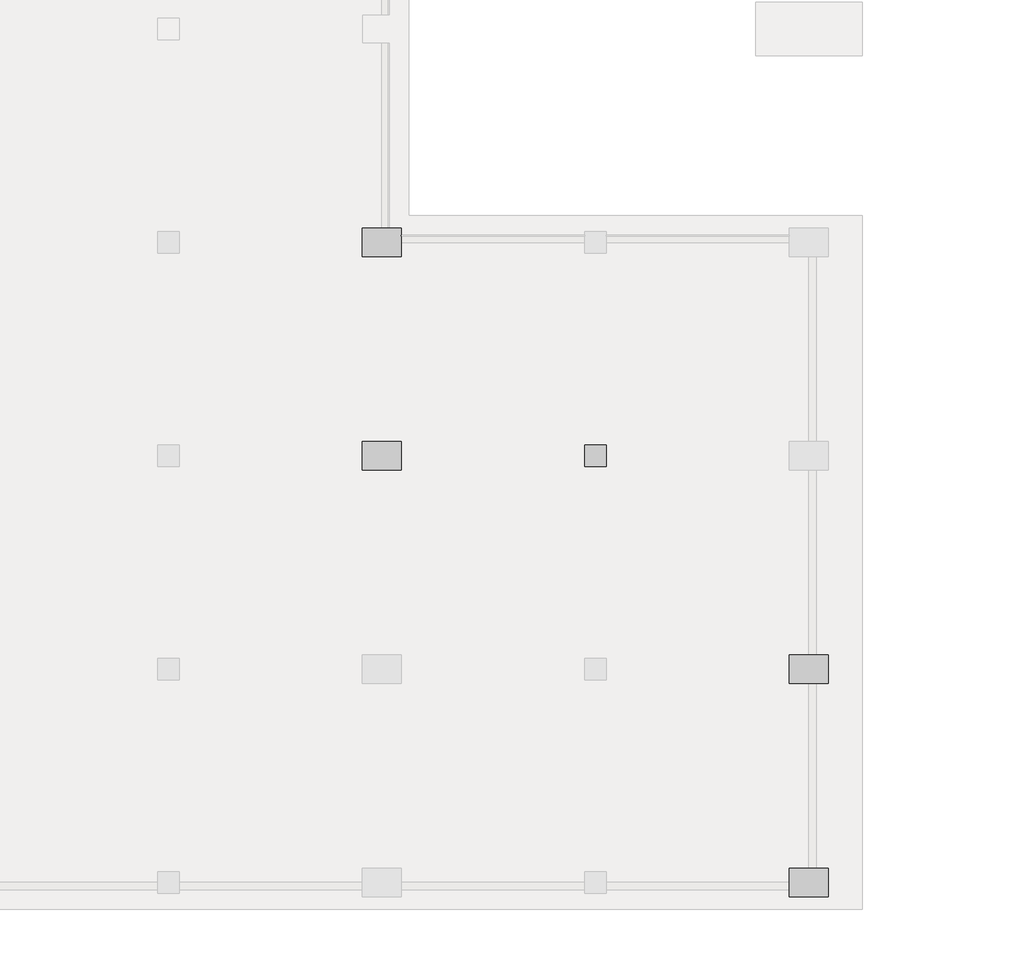
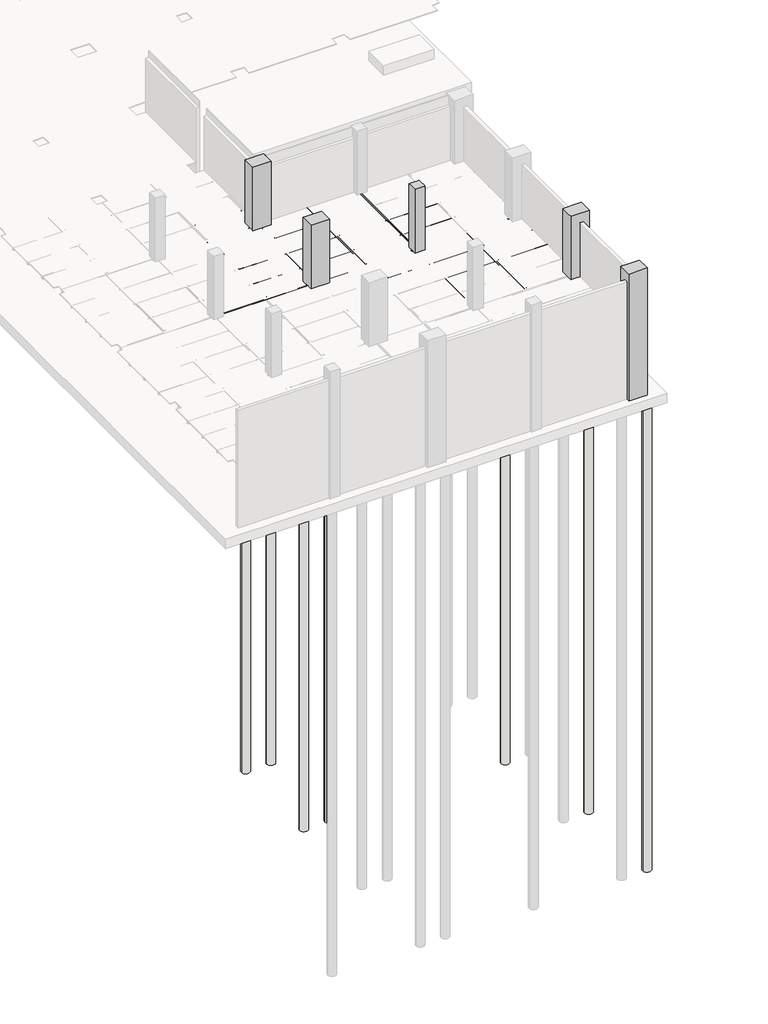
# Not in any storey, part 5 of 16: 26 beams, 7 slabs, 5 columns.
"""IFC4 building model written with IfcOpenShell, lengths in millimetres."""

from ifc_helpers import new_model, si_unit, point, frame, frame_2d, origin, place, context, project, spatial, polyline, circle_curve, trimmed, segment, composite_curve, outline, extrude, faceted_brep, element, save

model = new_model("IFC4")

# Units and contexts
model_context = context("Model", 3, world=origin())
ifc_project = project(units=[si_unit("LENGTHUNIT", "METRE", prefix="MILLI")], contexts=[model_context])

# Site, building
site = spatial("IfcSite", under=ifc_project)
building = spatial("IfcBuilding", under=site)

# Beams
placement = place(None, origin())
element("IfcBeam", 1, ObjectType="Steel Framing_H_KS : H_SB_AR_S02_H-400x200x8x13_BSG1", at=placement, inside=building, context=model_context, shape_type="SweptSolid", body=[
    extrude(outline(composite_curve([segment(polyline([(-47900.0, -4187.0381366), (-47900.0, -4200.0381366), (-48100.0, -4200.0381366), (-48100.0, -4187.0381366), (-48020.0, -4187.0381366)]), True, "CONTINUOUS"), segment(trimmed(circle_curve(frame_2d((-48020.0, -4171.0381366)), 16.0), [point((-48020.0, -4187.0381366))], [point((-48004.0, -4171.0381366))], True, "CARTESIAN"), True, "CONTINUOUS"), segment(polyline([(-48004.0, -4171.0381366), (-48004.0, -3829.0381366)]), True, "CONTINUOUS"), segment(trimmed(circle_curve(frame_2d((-48020.0, -3829.0381366)), 16.0), [point((-48004.0, -3829.0381366))], [point((-48020.0, -3813.0381366))], True, "CARTESIAN"), True, "CONTINUOUS"), segment(polyline([(-48020.0, -3813.0381366), (-48100.0, -3813.0381366), (-48100.0, -3800.0381366), (-47900.0, -3800.0381366), (-47900.0, -3813.0381366), (-47980.0, -3813.0381366)]), True, "CONTINUOUS"), segment(trimmed(circle_curve(frame_2d((-47980.0, -3829.0381366)), 16.0), [point((-47980.0, -3813.0381366))], [point((-47996.0, -3829.0381366))], True, "CARTESIAN"), True, "CONTINUOUS"), segment(polyline([(-47996.0, -3829.0381366), (-47996.0, -4171.0381366)]), True, "CONTINUOUS"), segment(trimmed(circle_curve(frame_2d((-47980.0, -4171.0381366)), 16.0), [point((-47996.0, -4171.0381366))], [point((-47980.0, -4187.0381366))], True, "CARTESIAN"), True, "CONTINUOUS"), segment(polyline([(-47980.0, -4187.0381366), (-47900.0, -4187.0381366)]), True, "CONTINUOUS")], self_intersect=False)), frame((30312.7, 0.0, 0.0), z_axis=(1.0, 0.0, 0.0), x_axis=(0.0, 1.0, 0.0)), (0.0, 0.0, 1.0), 5124.6),
])
element("IfcBeam", 2, ObjectType="Steel Framing_H_KS : H_SB_AR_S02_H-400x200x8x13_BSG2", at=placement, inside=building, context=model_context, shape_type="SweptSolid", body=[
    extrude(outline(composite_curve([segment(polyline([(-4187.0381366, 35900.0), (-4200.0381366, 35900.0), (-4200.0381366, 36100.0), (-4187.0381366, 36100.0), (-4187.0381366, 36020.0)]), True, "CONTINUOUS"), segment(trimmed(circle_curve(frame_2d((-4171.0381366, 36020.0)), 16.0), [point((-4187.0381366, 36020.0))], [point((-4171.0381366, 36004.0))], True, "CARTESIAN"), True, "CONTINUOUS"), segment(polyline([(-4171.0381366, 36004.0), (-3829.0381366, 36004.0)]), True, "CONTINUOUS"), segment(trimmed(circle_curve(frame_2d((-3829.0381366, 36020.0)), 16.0), [point((-3829.0381366, 36004.0))], [point((-3813.0381366, 36020.0))], True, "CARTESIAN"), True, "CONTINUOUS"), segment(polyline([(-3813.0381366, 36020.0), (-3813.0381366, 36100.0), (-3800.0381366, 36100.0), (-3800.0381366, 35900.0), (-3813.0381366, 35900.0), (-3813.0381366, 35980.0)]), True, "CONTINUOUS"), segment(trimmed(circle_curve(frame_2d((-3829.0381366, 35980.0)), 16.0), [point((-3813.0381366, 35980.0))], [point((-3829.0381366, 35996.0))], True, "CARTESIAN"), True, "CONTINUOUS"), segment(polyline([(-3829.0381366, 35996.0), (-4171.0381366, 35996.0)]), True, "CONTINUOUS"), segment(trimmed(circle_curve(frame_2d((-4171.0381366, 35980.0)), 16.0), [point((-4171.0381366, 35996.0))], [point((-4187.0381366, 35980.0))], True, "CARTESIAN"), True, "CONTINUOUS"), segment(polyline([(-4187.0381366, 35980.0), (-4187.0381366, 35900.0)]), True, "CONTINUOUS")], self_intersect=False)), frame((0.0, -47587.3, 0.0), z_axis=(0.0, 1.0, 0.0), x_axis=(0.0, 0.0, 1.0)), (0.0, 0.0, 1.0), 5174.6),
])
element("IfcBeam", 3, ObjectType="Steel Framing_H_KS : H_SB_AR_S02_H-400x200x8x13_BSB1", at=placement, inside=building, context=model_context, shape_type="SweptSolid", body=[
    extrude(outline(composite_curve([segment(polyline([(-4187.0381366, 32900.0), (-4200.0381366, 32900.0), (-4200.0381366, 33100.0), (-4187.0381366, 33100.0), (-4187.0381366, 33020.0)]), True, "CONTINUOUS"), segment(trimmed(circle_curve(frame_2d((-4171.0381366, 33020.0)), 16.0), [point((-4187.0381366, 33020.0))], [point((-4171.0381366, 33004.0))], True, "CARTESIAN"), True, "CONTINUOUS"), segment(polyline([(-4171.0381366, 33004.0), (-3829.0381366, 33004.0)]), True, "CONTINUOUS"), segment(trimmed(circle_curve(frame_2d((-3829.0381366, 33020.0)), 16.0), [point((-3829.0381366, 33004.0))], [point((-3813.0381366, 33020.0))], True, "CARTESIAN"), True, "CONTINUOUS"), segment(polyline([(-3813.0381366, 33020.0), (-3813.0381366, 33100.0), (-3800.0381366, 33100.0), (-3800.0381366, 32900.0), (-3813.0381366, 32900.0), (-3813.0381366, 32980.0)]), True, "CONTINUOUS"), segment(trimmed(circle_curve(frame_2d((-3829.0381366, 32980.0)), 16.0), [point((-3813.0381366, 32980.0))], [point((-3829.0381366, 32996.0))], True, "CARTESIAN"), True, "CONTINUOUS"), segment(polyline([(-3829.0381366, 32996.0), (-4171.0381366, 32996.0)]), True, "CONTINUOUS"), segment(trimmed(circle_curve(frame_2d((-4171.0381366, 32980.0)), 16.0), [point((-4171.0381366, 32996.0))], [point((-4187.0381366, 32980.0))], True, "CARTESIAN"), True, "CONTINUOUS"), segment(polyline([(-4187.0381366, 32980.0), (-4187.0381366, 32900.0)]), True, "CONTINUOUS")], self_intersect=False)), frame((0.0, -47887.3, 0.0), z_axis=(0.0, 1.0, 0.0), x_axis=(0.0, 0.0, 1.0)), (0.0, 0.0, 1.0), 5774.6),
])
element("IfcBeam", 4, ObjectType="Steel Framing_C_KS : H_SB_AR_S02_C-150x75x6.5x10_J1", at=placement, inside=building, context=model_context, shape_type="SweptSolid", body=[
    extrude(outline(composite_curve([segment(polyline([(-44977.2, -3800.0381366), (-44977.2, -3950.0381366), (-45052.2, -3950.0381366)]), True, "CONTINUOUS"), segment(trimmed(circle_curve(frame_2d((-45042.2, -3950.0381366)), 10.0), [point((-45052.2, -3950.0381366))], [point((-45042.2, -3940.0381366))], False, "CARTESIAN"), True, "CONTINUOUS"), segment(polyline([(-45042.2, -3940.0381366), (-44983.7, -3930.7726469), (-44983.7, -3819.3036264), (-45042.2, -3810.0381366)]), True, "CONTINUOUS"), segment(trimmed(circle_curve(frame_2d((-45042.2, -3800.0381366)), 10.0), [point((-45042.2, -3810.0381366))], [point((-45052.2, -3800.0381366))], False, "CARTESIAN"), True, "CONTINUOUS"), segment(polyline([(-45052.2, -3800.0381366), (-44977.2, -3800.0381366)]), True, "CONTINUOUS")], self_intersect=False)), frame((33112.7, 0.0, 0.0), z_axis=(1.0, 0.0, 0.0), x_axis=(0.0, 1.0, 0.0)), (0.0, 0.0, 1.0), 2774.6),
])
element("IfcBeam", 5, ObjectType="Steel Framing_C_KS : H_SB_AR_S02_C-150x75x6.5x10_J1", at=placement, inside=building, context=model_context, shape_type="SweptSolid", body=[
    extrude(outline(composite_curve([segment(polyline([(-46477.2, -3800.0381366), (-46477.2, -3950.0381366), (-46552.2, -3950.0381366)]), True, "CONTINUOUS"), segment(trimmed(circle_curve(frame_2d((-46542.2, -3950.0381366)), 10.0), [point((-46552.2, -3950.0381366))], [point((-46542.2, -3940.0381366))], False, "CARTESIAN"), True, "CONTINUOUS"), segment(polyline([(-46542.2, -3940.0381366), (-46483.7, -3930.7726469), (-46483.7, -3819.3036264), (-46542.2, -3810.0381366)]), True, "CONTINUOUS"), segment(trimmed(circle_curve(frame_2d((-46542.2, -3800.0381366)), 10.0), [point((-46542.2, -3810.0381366))], [point((-46552.2, -3800.0381366))], False, "CARTESIAN"), True, "CONTINUOUS"), segment(polyline([(-46552.2, -3800.0381366), (-46477.2, -3800.0381366)]), True, "CONTINUOUS")], self_intersect=False)), frame((33112.7, 0.0, 0.0), z_axis=(1.0, 0.0, 0.0), x_axis=(0.0, 1.0, 0.0)), (0.0, 0.0, 1.0), 2774.6),
])
element("IfcBeam", 6, ObjectType="Steel Framing_C_KS : H_SB_AR_S02_C-150x75x6.5x10_J1", at=placement, inside=building, context=model_context, shape_type="SweptSolid", body=[
    extrude(outline(composite_curve([segment(polyline([(-43477.2, -3800.0381366), (-43477.2, -3950.0381366), (-43552.2, -3950.0381366)]), True, "CONTINUOUS"), segment(trimmed(circle_curve(frame_2d((-43542.2, -3950.0381366)), 10.0), [point((-43552.2, -3950.0381366))], [point((-43542.2, -3940.0381366))], False, "CARTESIAN"), True, "CONTINUOUS"), segment(polyline([(-43542.2, -3940.0381366), (-43483.7, -3930.7726469), (-43483.7, -3819.3036264), (-43542.2, -3810.0381366)]), True, "CONTINUOUS"), segment(trimmed(circle_curve(frame_2d((-43542.2, -3800.0381366)), 10.0), [point((-43542.2, -3810.0381366))], [point((-43552.2, -3800.0381366))], False, "CARTESIAN"), True, "CONTINUOUS"), segment(polyline([(-43552.2, -3800.0381366), (-43477.2, -3800.0381366)]), True, "CONTINUOUS")], self_intersect=False)), frame((33112.7, 0.0, 0.0), z_axis=(1.0, 0.0, 0.0), x_axis=(0.0, 1.0, 0.0)), (0.0, 0.0, 1.0), 2774.6),
])
element("IfcBeam", 7, ObjectType="Steel Framing_H_KS : H_SB_AR_S02_H-400x200x8x13_BSG1", at=placement, inside=building, context=model_context, shape_type="SweptSolid", body=[
    extrude(outline(composite_curve([segment(polyline([(-47900.0, -4187.0381366), (-47900.0, -4200.0381366), (-48100.0, -4200.0381366), (-48100.0, -4187.0381366), (-48020.0, -4187.0381366)]), True, "CONTINUOUS"), segment(trimmed(circle_curve(frame_2d((-48020.0, -4171.0381366)), 16.0), [point((-48020.0, -4187.0381366))], [point((-48004.0, -4171.0381366))], True, "CARTESIAN"), True, "CONTINUOUS"), segment(polyline([(-48004.0, -4171.0381366), (-48004.0, -3829.0381366)]), True, "CONTINUOUS"), segment(trimmed(circle_curve(frame_2d((-48020.0, -3829.0381366)), 16.0), [point((-48004.0, -3829.0381366))], [point((-48020.0, -3813.0381366))], True, "CARTESIAN"), True, "CONTINUOUS"), segment(polyline([(-48020.0, -3813.0381366), (-48100.0, -3813.0381366), (-48100.0, -3800.0381366), (-47900.0, -3800.0381366), (-47900.0, -3813.0381366), (-47980.0, -3813.0381366)]), True, "CONTINUOUS"), segment(trimmed(circle_curve(frame_2d((-47980.0, -3829.0381366)), 16.0), [point((-47980.0, -3813.0381366))], [point((-47996.0, -3829.0381366))], True, "CARTESIAN"), True, "CONTINUOUS"), segment(polyline([(-47996.0, -3829.0381366), (-47996.0, -4171.0381366)]), True, "CONTINUOUS"), segment(trimmed(circle_curve(frame_2d((-47980.0, -4171.0381366)), 16.0), [point((-47996.0, -4171.0381366))], [point((-47980.0, -4187.0381366))], True, "CARTESIAN"), True, "CONTINUOUS"), segment(polyline([(-47980.0, -4187.0381366), (-47900.0, -4187.0381366)]), True, "CONTINUOUS")], self_intersect=False)), frame((36562.7, 0.0, 0.0), z_axis=(1.0, 0.0, 0.0), x_axis=(0.0, 1.0, 0.0)), (0.0, 0.0, 1.0), 5124.6),
])
element("IfcBeam", 8, ObjectType="Steel Framing_H_KS : H_SB_AR_S02_H-400x200x8x13_BSG2", at=placement, inside=building, context=model_context, shape_type="SweptSolid", body=[
    extrude(outline(composite_curve([segment(polyline([(-4187.0381366, 41900.0), (-4200.0381366, 41900.0), (-4200.0381366, 42100.0), (-4187.0381366, 42100.0), (-4187.0381366, 42020.0)]), True, "CONTINUOUS"), segment(trimmed(circle_curve(frame_2d((-4171.0381366, 42020.0)), 16.0), [point((-4187.0381366, 42020.0))], [point((-4171.0381366, 42004.0))], True, "CARTESIAN"), True, "CONTINUOUS"), segment(polyline([(-4171.0381366, 42004.0), (-3829.0381366, 42004.0)]), True, "CONTINUOUS"), segment(trimmed(circle_curve(frame_2d((-3829.0381366, 42020.0)), 16.0), [point((-3829.0381366, 42004.0))], [point((-3813.0381366, 42020.0))], True, "CARTESIAN"), True, "CONTINUOUS"), segment(polyline([(-3813.0381366, 42020.0), (-3813.0381366, 42100.0), (-3800.0381366, 42100.0), (-3800.0381366, 41900.0), (-3813.0381366, 41900.0), (-3813.0381366, 41980.0)]), True, "CONTINUOUS"), segment(trimmed(circle_curve(frame_2d((-3829.0381366, 41980.0)), 16.0), [point((-3813.0381366, 41980.0))], [point((-3829.0381366, 41996.0))], True, "CARTESIAN"), True, "CONTINUOUS"), segment(polyline([(-3829.0381366, 41996.0), (-4171.0381366, 41996.0)]), True, "CONTINUOUS"), segment(trimmed(circle_curve(frame_2d((-4171.0381366, 41980.0)), 16.0), [point((-4171.0381366, 41996.0))], [point((-4187.0381366, 41980.0))], True, "CARTESIAN"), True, "CONTINUOUS"), segment(polyline([(-4187.0381366, 41980.0), (-4187.0381366, 41900.0)]), True, "CONTINUOUS")], self_intersect=False)), frame((0.0, -47687.3, 0.0), z_axis=(0.0, 1.0, 0.0), x_axis=(0.0, 0.0, 1.0)), (0.0, 0.0, 1.0), 5374.6),
])
element("IfcBeam", 9, ObjectType="Steel Framing_H_KS : H_SB_AR_S02_H-400x200x8x13_BSB1", at=placement, inside=building, context=model_context, shape_type="SweptSolid", body=[
    extrude(outline(composite_curve([segment(polyline([(-4187.0381366, 38900.0), (-4200.0381366, 38900.0), (-4200.0381366, 39100.0), (-4187.0381366, 39100.0), (-4187.0381366, 39020.0)]), True, "CONTINUOUS"), segment(trimmed(circle_curve(frame_2d((-4171.0381366, 39020.0)), 16.0), [point((-4187.0381366, 39020.0))], [point((-4171.0381366, 39004.0))], True, "CARTESIAN"), True, "CONTINUOUS"), segment(polyline([(-4171.0381366, 39004.0), (-3829.0381366, 39004.0)]), True, "CONTINUOUS"), segment(trimmed(circle_curve(frame_2d((-3829.0381366, 39020.0)), 16.0), [point((-3829.0381366, 39004.0))], [point((-3813.0381366, 39020.0))], True, "CARTESIAN"), True, "CONTINUOUS"), segment(polyline([(-3813.0381366, 39020.0), (-3813.0381366, 39100.0), (-3800.0381366, 39100.0), (-3800.0381366, 38900.0), (-3813.0381366, 38900.0), (-3813.0381366, 38980.0)]), True, "CONTINUOUS"), segment(trimmed(circle_curve(frame_2d((-3829.0381366, 38980.0)), 16.0), [point((-3813.0381366, 38980.0))], [point((-3829.0381366, 38996.0))], True, "CARTESIAN"), True, "CONTINUOUS"), segment(polyline([(-3829.0381366, 38996.0), (-4171.0381366, 38996.0)]), True, "CONTINUOUS"), segment(trimmed(circle_curve(frame_2d((-4171.0381366, 38980.0)), 16.0), [point((-4171.0381366, 38996.0))], [point((-4187.0381366, 38980.0))], True, "CARTESIAN"), True, "CONTINUOUS"), segment(polyline([(-4187.0381366, 38980.0), (-4187.0381366, 38900.0)]), True, "CONTINUOUS")], self_intersect=False)), frame((0.0, -47887.3, 0.0), z_axis=(0.0, 1.0, 0.0), x_axis=(0.0, 0.0, 1.0)), (0.0, 0.0, 1.0), 5887.3),
])
element("IfcBeam", 10, ObjectType="Steel Framing_C_KS : H_SB_AR_S02_C-150x75x6.5x10_J1", at=placement, inside=building, context=model_context, shape_type="SweptSolid", body=[
    extrude(outline(composite_curve([segment(polyline([(-44977.2, -3800.0381366), (-44977.2, -3950.0381366), (-45052.2, -3950.0381366)]), True, "CONTINUOUS"), segment(trimmed(circle_curve(frame_2d((-45042.2, -3950.0381366)), 10.0), [point((-45052.2, -3950.0381366))], [point((-45042.2, -3940.0381366))], False, "CARTESIAN"), True, "CONTINUOUS"), segment(polyline([(-45042.2, -3940.0381366), (-44983.7, -3930.7726469), (-44983.7, -3819.3036264), (-45042.2, -3810.0381366)]), True, "CONTINUOUS"), segment(trimmed(circle_curve(frame_2d((-45042.2, -3800.0381366)), 10.0), [point((-45042.2, -3810.0381366))], [point((-45052.2, -3800.0381366))], False, "CARTESIAN"), True, "CONTINUOUS"), segment(polyline([(-45052.2, -3800.0381366), (-44977.2, -3800.0381366)]), True, "CONTINUOUS")], self_intersect=False)), frame((36112.7, 0.0, 0.0), z_axis=(1.0, 0.0, 0.0), x_axis=(0.0, 1.0, 0.0)), (0.0, 0.0, 1.0), 2774.6),
])
element("IfcBeam", 11, ObjectType="Steel Framing_C_KS : H_SB_AR_S02_C-150x75x6.5x10_J1", at=placement, inside=building, context=model_context, shape_type="SweptSolid", body=[
    extrude(outline(composite_curve([segment(polyline([(-46477.2, -3800.0381366), (-46477.2, -3950.0381366), (-46552.2, -3950.0381366)]), True, "CONTINUOUS"), segment(trimmed(circle_curve(frame_2d((-46542.2, -3950.0381366)), 10.0), [point((-46552.2, -3950.0381366))], [point((-46542.2, -3940.0381366))], False, "CARTESIAN"), True, "CONTINUOUS"), segment(polyline([(-46542.2, -3940.0381366), (-46483.7, -3930.7726469), (-46483.7, -3819.3036264), (-46542.2, -3810.0381366)]), True, "CONTINUOUS"), segment(trimmed(circle_curve(frame_2d((-46542.2, -3800.0381366)), 10.0), [point((-46542.2, -3810.0381366))], [point((-46552.2, -3800.0381366))], False, "CARTESIAN"), True, "CONTINUOUS"), segment(polyline([(-46552.2, -3800.0381366), (-46477.2, -3800.0381366)]), True, "CONTINUOUS")], self_intersect=False)), frame((36112.7, 0.0, 0.0), z_axis=(1.0, 0.0, 0.0), x_axis=(0.0, 1.0, 0.0)), (0.0, 0.0, 1.0), 2774.6),
])
element("IfcBeam", 12, ObjectType="Steel Framing_C_KS : H_SB_AR_S02_C-150x75x6.5x10_J1", at=placement, inside=building, context=model_context, shape_type="SweptSolid", body=[
    extrude(outline(composite_curve([segment(polyline([(-43477.2, -3800.0381366), (-43477.2, -3950.0381366), (-43552.2, -3950.0381366)]), True, "CONTINUOUS"), segment(trimmed(circle_curve(frame_2d((-43542.2, -3950.0381366)), 10.0), [point((-43552.2, -3950.0381366))], [point((-43542.2, -3940.0381366))], False, "CARTESIAN"), True, "CONTINUOUS"), segment(polyline([(-43542.2, -3940.0381366), (-43483.7, -3930.7726469), (-43483.7, -3819.3036264), (-43542.2, -3810.0381366)]), True, "CONTINUOUS"), segment(trimmed(circle_curve(frame_2d((-43542.2, -3800.0381366)), 10.0), [point((-43542.2, -3810.0381366))], [point((-43552.2, -3800.0381366))], False, "CARTESIAN"), True, "CONTINUOUS"), segment(polyline([(-43552.2, -3800.0381366), (-43477.2, -3800.0381366)]), True, "CONTINUOUS")], self_intersect=False)), frame((36112.7, 0.0, 0.0), z_axis=(1.0, 0.0, 0.0), x_axis=(0.0, 1.0, 0.0)), (0.0, 0.0, 1.0), 2774.6),
])
element("IfcBeam", 13, ObjectType="Steel Framing_C_KS : H_SB_AR_S02_C-150x75x6.5x10_J1", at=placement, inside=building, context=model_context, shape_type="SweptSolid", body=[
    extrude(outline(composite_curve([segment(polyline([(-44977.2, -3800.0381366), (-44977.2, -3950.0381366), (-45052.2, -3950.0381366)]), True, "CONTINUOUS"), segment(trimmed(circle_curve(frame_2d((-45042.2, -3950.0381366)), 10.0), [point((-45052.2, -3950.0381366))], [point((-45042.2, -3940.0381366))], False, "CARTESIAN"), True, "CONTINUOUS"), segment(polyline([(-45042.2, -3940.0381366), (-44983.7, -3930.7726469), (-44983.7, -3819.3036264), (-45042.2, -3810.0381366)]), True, "CONTINUOUS"), segment(trimmed(circle_curve(frame_2d((-45042.2, -3800.0381366)), 10.0), [point((-45042.2, -3810.0381366))], [point((-45052.2, -3800.0381366))], False, "CARTESIAN"), True, "CONTINUOUS"), segment(polyline([(-45052.2, -3800.0381366), (-44977.2, -3800.0381366)]), True, "CONTINUOUS")], self_intersect=False)), frame((39112.7, 0.0, 0.0), z_axis=(1.0, 0.0, 0.0), x_axis=(0.0, 1.0, 0.0)), (0.0, 0.0, 1.0), 2774.6),
])
element("IfcBeam", 14, ObjectType="Steel Framing_C_KS : H_SB_AR_S02_C-150x75x6.5x10_J1", at=placement, inside=building, context=model_context, shape_type="SweptSolid", body=[
    extrude(outline(composite_curve([segment(polyline([(-46477.2, -3800.0381366), (-46477.2, -3950.0381366), (-46552.2, -3950.0381366)]), True, "CONTINUOUS"), segment(trimmed(circle_curve(frame_2d((-46542.2, -3950.0381366)), 10.0), [point((-46552.2, -3950.0381366))], [point((-46542.2, -3940.0381366))], False, "CARTESIAN"), True, "CONTINUOUS"), segment(polyline([(-46542.2, -3940.0381366), (-46483.7, -3930.7726469), (-46483.7, -3819.3036264), (-46542.2, -3810.0381366)]), True, "CONTINUOUS"), segment(trimmed(circle_curve(frame_2d((-46542.2, -3800.0381366)), 10.0), [point((-46542.2, -3810.0381366))], [point((-46552.2, -3800.0381366))], False, "CARTESIAN"), True, "CONTINUOUS"), segment(polyline([(-46552.2, -3800.0381366), (-46477.2, -3800.0381366)]), True, "CONTINUOUS")], self_intersect=False)), frame((39112.7, 0.0, 0.0), z_axis=(1.0, 0.0, 0.0), x_axis=(0.0, 1.0, 0.0)), (0.0, 0.0, 1.0), 2774.6),
])
element("IfcBeam", 15, ObjectType="Steel Framing_H_KS : H_SB_AR_S02_H-400x200x8x13_BSG1", at=placement, inside=building, context=model_context, shape_type="SweptSolid", body=[
    extrude(outline(composite_curve([segment(polyline([(-47900.0, -4187.0381366), (-47900.0, -4200.0381366), (-48100.0, -4200.0381366), (-48100.0, -4187.0381366), (-48020.0, -4187.0381366)]), True, "CONTINUOUS"), segment(trimmed(circle_curve(frame_2d((-48020.0, -4171.0381366)), 16.0), [point((-48020.0, -4187.0381366))], [point((-48004.0, -4171.0381366))], True, "CARTESIAN"), True, "CONTINUOUS"), segment(polyline([(-48004.0, -4171.0381366), (-48004.0, -3829.0381366)]), True, "CONTINUOUS"), segment(trimmed(circle_curve(frame_2d((-48020.0, -3829.0381366)), 16.0), [point((-48004.0, -3829.0381366))], [point((-48020.0, -3813.0381366))], True, "CARTESIAN"), True, "CONTINUOUS"), segment(polyline([(-48020.0, -3813.0381366), (-48100.0, -3813.0381366), (-48100.0, -3800.0381366), (-47900.0, -3800.0381366), (-47900.0, -3813.0381366), (-47980.0, -3813.0381366)]), True, "CONTINUOUS"), segment(trimmed(circle_curve(frame_2d((-47980.0, -3829.0381366)), 16.0), [point((-47980.0, -3813.0381366))], [point((-47996.0, -3829.0381366))], True, "CARTESIAN"), True, "CONTINUOUS"), segment(polyline([(-47996.0, -3829.0381366), (-47996.0, -4171.0381366)]), True, "CONTINUOUS"), segment(trimmed(circle_curve(frame_2d((-47980.0, -4171.0381366)), 16.0), [point((-47996.0, -4171.0381366))], [point((-47980.0, -4187.0381366))], True, "CARTESIAN"), True, "CONTINUOUS"), segment(polyline([(-47980.0, -4187.0381366), (-47900.0, -4187.0381366)]), True, "CONTINUOUS")], self_intersect=False)), frame((42312.7, 0.0, 0.0), z_axis=(1.0, 0.0, 0.0), x_axis=(0.0, 1.0, 0.0)), (0.0, 0.0, 1.0), 5124.6),
])
element("IfcBeam", 16, ObjectType="Steel Framing_C_KS : H_SB_AR_S02_C-150x75x6.5x10_J1", at=placement, inside=building, context=model_context, shape_type="SweptSolid", body=[
    extrude(outline(composite_curve([segment(polyline([(-44977.2, -3800.0381366), (-44977.2, -3950.0381366), (-45052.2, -3950.0381366)]), True, "CONTINUOUS"), segment(trimmed(circle_curve(frame_2d((-45042.2, -3950.0381366)), 10.0), [point((-45052.2, -3950.0381366))], [point((-45042.2, -3940.0381366))], False, "CARTESIAN"), True, "CONTINUOUS"), segment(polyline([(-45042.2, -3940.0381366), (-44983.7, -3930.7726469), (-44983.7, -3819.3036264), (-45042.2, -3810.0381366)]), True, "CONTINUOUS"), segment(trimmed(circle_curve(frame_2d((-45042.2, -3800.0381366)), 10.0), [point((-45042.2, -3810.0381366))], [point((-45052.2, -3800.0381366))], False, "CARTESIAN"), True, "CONTINUOUS"), segment(polyline([(-45052.2, -3800.0381366), (-44977.2, -3800.0381366)]), True, "CONTINUOUS")], self_intersect=False)), frame((42112.7, 0.0, 0.0), z_axis=(1.0, 0.0, 0.0), x_axis=(0.0, 1.0, 0.0)), (0.0, 0.0, 1.0), 2774.6),
])
element("IfcBeam", 17, ObjectType="Steel Framing_C_KS : H_SB_AR_S02_C-150x75x6.5x10_J1", at=placement, inside=building, context=model_context, shape_type="SweptSolid", body=[
    extrude(outline(composite_curve([segment(polyline([(-46477.2, -3800.0381366), (-46477.2, -3950.0381366), (-46552.2, -3950.0381366)]), True, "CONTINUOUS"), segment(trimmed(circle_curve(frame_2d((-46542.2, -3950.0381366)), 10.0), [point((-46552.2, -3950.0381366))], [point((-46542.2, -3940.0381366))], False, "CARTESIAN"), True, "CONTINUOUS"), segment(polyline([(-46542.2, -3940.0381366), (-46483.7, -3930.7726469), (-46483.7, -3819.3036264), (-46542.2, -3810.0381366)]), True, "CONTINUOUS"), segment(trimmed(circle_curve(frame_2d((-46542.2, -3800.0381366)), 10.0), [point((-46542.2, -3810.0381366))], [point((-46552.2, -3800.0381366))], False, "CARTESIAN"), True, "CONTINUOUS"), segment(polyline([(-46552.2, -3800.0381366), (-46477.2, -3800.0381366)]), True, "CONTINUOUS")], self_intersect=False)), frame((42112.7, 0.0, 0.0), z_axis=(1.0, 0.0, 0.0), x_axis=(0.0, 1.0, 0.0)), (0.0, 0.0, 1.0), 2774.6),
])
element("IfcBeam", 18, ObjectType="Steel Framing_H_KS : H_SB_AR_S02_H-400x200x8x13_BSG2", at=placement, inside=building, context=model_context, shape_type="SweptSolid", body=[
    extrude(outline(composite_curve([segment(polyline([(-4187.0381366, 41900.0), (-4200.0381366, 41900.0), (-4200.0381366, 42100.0), (-4187.0381366, 42100.0), (-4187.0381366, 42020.0)]), True, "CONTINUOUS"), segment(trimmed(circle_curve(frame_2d((-4171.0381366, 42020.0)), 16.0), [point((-4187.0381366, 42020.0))], [point((-4171.0381366, 42004.0))], True, "CARTESIAN"), True, "CONTINUOUS"), segment(polyline([(-4171.0381366, 42004.0), (-3829.0381366, 42004.0)]), True, "CONTINUOUS"), segment(trimmed(circle_curve(frame_2d((-3829.0381366, 42020.0)), 16.0), [point((-3829.0381366, 42004.0))], [point((-3813.0381366, 42020.0))], True, "CARTESIAN"), True, "CONTINUOUS"), segment(polyline([(-3813.0381366, 42020.0), (-3813.0381366, 42100.0), (-3800.0381366, 42100.0), (-3800.0381366, 41900.0), (-3813.0381366, 41900.0), (-3813.0381366, 41980.0)]), True, "CONTINUOUS"), segment(trimmed(circle_curve(frame_2d((-3829.0381366, 41980.0)), 16.0), [point((-3813.0381366, 41980.0))], [point((-3829.0381366, 41996.0))], True, "CARTESIAN"), True, "CONTINUOUS"), segment(polyline([(-3829.0381366, 41996.0), (-4171.0381366, 41996.0)]), True, "CONTINUOUS"), segment(trimmed(circle_curve(frame_2d((-4171.0381366, 41980.0)), 16.0), [point((-4171.0381366, 41996.0))], [point((-4187.0381366, 41980.0))], True, "CARTESIAN"), True, "CONTINUOUS"), segment(polyline([(-4187.0381366, 41980.0), (-4187.0381366, 41900.0)]), True, "CONTINUOUS")], self_intersect=False)), frame((0.0, -53687.3, 0.0), z_axis=(0.0, 1.0, 0.0), x_axis=(0.0, 0.0, 1.0)), (0.0, 0.0, 1.0), 5374.6),
])
element("IfcBeam", 19, ObjectType="Steel Framing_C_KS : H_SB_AR_S02_C-150x75x6.5x10_J1", at=placement, inside=building, context=model_context, shape_type="SweptSolid", body=[
    extrude(outline(composite_curve([segment(polyline([(-49477.2, -3800.0381366), (-49477.2, -3950.0381366), (-49552.2, -3950.0381366)]), True, "CONTINUOUS"), segment(trimmed(circle_curve(frame_2d((-49542.2, -3950.0381366)), 10.0), [point((-49552.2, -3950.0381366))], [point((-49542.2, -3940.0381366))], False, "CARTESIAN"), True, "CONTINUOUS"), segment(polyline([(-49542.2, -3940.0381366), (-49483.7, -3930.7726469), (-49483.7, -3819.3036264), (-49542.2, -3810.0381366)]), True, "CONTINUOUS"), segment(trimmed(circle_curve(frame_2d((-49542.2, -3800.0381366)), 10.0), [point((-49542.2, -3810.0381366))], [point((-49552.2, -3800.0381366))], False, "CARTESIAN"), True, "CONTINUOUS"), segment(polyline([(-49552.2, -3800.0381366), (-49477.2, -3800.0381366)]), True, "CONTINUOUS")], self_intersect=False)), frame((39112.7, 0.0, 0.0), z_axis=(1.0, 0.0, 0.0), x_axis=(0.0, 1.0, 0.0)), (0.0, 0.0, 1.0), 2774.6),
])
element("IfcBeam", 20, ObjectType="Steel Framing_H_KS : H_SB_AR_S02_H-400x200x8x13_BSB1", at=placement, inside=building, context=model_context, shape_type="SweptSolid", body=[
    extrude(outline(composite_curve([segment(polyline([(-4187.0381366, 44900.0), (-4200.0381366, 44900.0), (-4200.0381366, 45100.0), (-4187.0381366, 45100.0), (-4187.0381366, 45020.0)]), True, "CONTINUOUS"), segment(trimmed(circle_curve(frame_2d((-4171.0381366, 45020.0)), 16.0), [point((-4187.0381366, 45020.0))], [point((-4171.0381366, 45004.0))], True, "CARTESIAN"), True, "CONTINUOUS"), segment(polyline([(-4171.0381366, 45004.0), (-3829.0381366, 45004.0)]), True, "CONTINUOUS"), segment(trimmed(circle_curve(frame_2d((-3829.0381366, 45020.0)), 16.0), [point((-3829.0381366, 45004.0))], [point((-3813.0381366, 45020.0))], True, "CARTESIAN"), True, "CONTINUOUS"), segment(polyline([(-3813.0381366, 45020.0), (-3813.0381366, 45100.0), (-3800.0381366, 45100.0), (-3800.0381366, 44900.0), (-3813.0381366, 44900.0), (-3813.0381366, 44980.0)]), True, "CONTINUOUS"), segment(trimmed(circle_curve(frame_2d((-3829.0381366, 44980.0)), 16.0), [point((-3813.0381366, 44980.0))], [point((-3829.0381366, 44996.0))], True, "CARTESIAN"), True, "CONTINUOUS"), segment(polyline([(-3829.0381366, 44996.0), (-4171.0381366, 44996.0)]), True, "CONTINUOUS"), segment(trimmed(circle_curve(frame_2d((-4171.0381366, 44980.0)), 16.0), [point((-4171.0381366, 44996.0))], [point((-4187.0381366, 44980.0))], True, "CARTESIAN"), True, "CONTINUOUS"), segment(polyline([(-4187.0381366, 44980.0), (-4187.0381366, 44900.0)]), True, "CONTINUOUS")], self_intersect=False)), frame((0.0, -53887.3, 0.0), z_axis=(0.0, 1.0, 0.0), x_axis=(0.0, 0.0, 1.0)), (0.0, 0.0, 1.0), 5774.6),
])
element("IfcBeam", 21, ObjectType="Steel Framing_C_KS : H_SB_AR_S02_C-150x75x6.5x10_J1", at=placement, inside=building, context=model_context, shape_type="SweptSolid", body=[
    extrude(outline(composite_curve([segment(polyline([(-50977.2, -3800.0381366), (-50977.2, -3950.0381366), (-51052.2, -3950.0381366)]), True, "CONTINUOUS"), segment(trimmed(circle_curve(frame_2d((-51042.2, -3950.0381366)), 10.0), [point((-51052.2, -3950.0381366))], [point((-51042.2, -3940.0381366))], False, "CARTESIAN"), True, "CONTINUOUS"), segment(polyline([(-51042.2, -3940.0381366), (-50983.7, -3930.7726469), (-50983.7, -3819.3036264), (-51042.2, -3810.0381366)]), True, "CONTINUOUS"), segment(trimmed(circle_curve(frame_2d((-51042.2, -3800.0381366)), 10.0), [point((-51042.2, -3810.0381366))], [point((-51052.2, -3800.0381366))], False, "CARTESIAN"), True, "CONTINUOUS"), segment(polyline([(-51052.2, -3800.0381366), (-50977.2, -3800.0381366)]), True, "CONTINUOUS")], self_intersect=False)), frame((42112.7, 0.0, 0.0), z_axis=(1.0, 0.0, 0.0), x_axis=(0.0, 1.0, 0.0)), (0.0, 0.0, 1.0), 2774.6),
])
element("IfcBeam", 22, ObjectType="Steel Framing_C_KS : H_SB_AR_S02_C-150x75x6.5x10_J1", at=placement, inside=building, context=model_context, shape_type="SweptSolid", body=[
    extrude(outline(composite_curve([segment(polyline([(-49477.2, -3800.0381366), (-49477.2, -3950.0381366), (-49552.2, -3950.0381366)]), True, "CONTINUOUS"), segment(trimmed(circle_curve(frame_2d((-49542.2, -3950.0381366)), 10.0), [point((-49552.2, -3950.0381366))], [point((-49542.2, -3940.0381366))], False, "CARTESIAN"), True, "CONTINUOUS"), segment(polyline([(-49542.2, -3940.0381366), (-49483.7, -3930.7726469), (-49483.7, -3819.3036264), (-49542.2, -3810.0381366)]), True, "CONTINUOUS"), segment(trimmed(circle_curve(frame_2d((-49542.2, -3800.0381366)), 10.0), [point((-49542.2, -3810.0381366))], [point((-49552.2, -3800.0381366))], False, "CARTESIAN"), True, "CONTINUOUS"), segment(polyline([(-49552.2, -3800.0381366), (-49477.2, -3800.0381366)]), True, "CONTINUOUS")], self_intersect=False)), frame((42112.7, 0.0, 0.0), z_axis=(1.0, 0.0, 0.0), x_axis=(0.0, 1.0, 0.0)), (0.0, 0.0, 1.0), 2774.6),
])
element("IfcBeam", 23, ObjectType="Steel Framing_C_KS : H_SB_AR_S02_C-150x75x6.5x10_J1", at=placement, inside=building, context=model_context, shape_type="SweptSolid", body=[
    extrude(outline(composite_curve([segment(polyline([(-50977.2, -3800.0381366), (-50977.2, -3950.0381366), (-51052.2, -3950.0381366)]), True, "CONTINUOUS"), segment(trimmed(circle_curve(frame_2d((-51042.2, -3950.0381366)), 10.0), [point((-51052.2, -3950.0381366))], [point((-51042.2, -3940.0381366))], False, "CARTESIAN"), True, "CONTINUOUS"), segment(polyline([(-51042.2, -3940.0381366), (-50983.7, -3930.7726469), (-50983.7, -3819.3036264), (-51042.2, -3810.0381366)]), True, "CONTINUOUS"), segment(trimmed(circle_curve(frame_2d((-51042.2, -3800.0381366)), 10.0), [point((-51042.2, -3810.0381366))], [point((-51052.2, -3800.0381366))], False, "CARTESIAN"), True, "CONTINUOUS"), segment(polyline([(-51052.2, -3800.0381366), (-50977.2, -3800.0381366)]), True, "CONTINUOUS")], self_intersect=False)), frame((45112.7, 0.0, 0.0), z_axis=(1.0, 0.0, 0.0), x_axis=(0.0, 1.0, 0.0)), (0.0, 0.0, 1.0), 2887.3),
])
element("IfcBeam", 24, ObjectType="Steel Framing_C_KS : H_SB_AR_S02_C-150x75x6.5x10_J1", at=placement, inside=building, context=model_context, shape_type="SweptSolid", body=[
    extrude(outline(composite_curve([segment(polyline([(-49477.2, -3800.0381366), (-49477.2, -3950.0381366), (-49552.2, -3950.0381366)]), True, "CONTINUOUS"), segment(trimmed(circle_curve(frame_2d((-49542.2, -3950.0381366)), 10.0), [point((-49552.2, -3950.0381366))], [point((-49542.2, -3940.0381366))], False, "CARTESIAN"), True, "CONTINUOUS"), segment(polyline([(-49542.2, -3940.0381366), (-49483.7, -3930.7726469), (-49483.7, -3819.3036264), (-49542.2, -3810.0381366)]), True, "CONTINUOUS"), segment(trimmed(circle_curve(frame_2d((-49542.2, -3800.0381366)), 10.0), [point((-49542.2, -3810.0381366))], [point((-49552.2, -3800.0381366))], False, "CARTESIAN"), True, "CONTINUOUS"), segment(polyline([(-49552.2, -3800.0381366), (-49477.2, -3800.0381366)]), True, "CONTINUOUS")], self_intersect=False)), frame((45112.7, 0.0, 0.0), z_axis=(1.0, 0.0, 0.0), x_axis=(0.0, 1.0, 0.0)), (0.0, 0.0, 1.0), 2887.3),
])
element("IfcBeam", 25, ObjectType="Steel Framing_H_KS : H_SB_AR_S02_H-400x200x8x13_BSG1", at=placement, inside=building, context=model_context, shape_type="SweptSolid", body=[
    extrude(outline(composite_curve([segment(polyline([(-41900.0, -4187.0381366), (-41900.0, -4200.0381366), (-42100.0, -4200.0381366), (-42100.0, -4187.0381366), (-42020.0, -4187.0381366)]), True, "CONTINUOUS"), segment(trimmed(circle_curve(frame_2d((-42020.0, -4171.0381366)), 16.0), [point((-42020.0, -4187.0381366))], [point((-42004.0, -4171.0381366))], True, "CARTESIAN"), True, "CONTINUOUS"), segment(polyline([(-42004.0, -4171.0381366), (-42004.0, -3829.0381366)]), True, "CONTINUOUS"), segment(trimmed(circle_curve(frame_2d((-42020.0, -3829.0381366)), 16.0), [point((-42004.0, -3829.0381366))], [point((-42020.0, -3813.0381366))], True, "CARTESIAN"), True, "CONTINUOUS"), segment(polyline([(-42020.0, -3813.0381366), (-42100.0, -3813.0381366), (-42100.0, -3800.0381366), (-41900.0, -3800.0381366), (-41900.0, -3813.0381366), (-41980.0, -3813.0381366)]), True, "CONTINUOUS"), segment(trimmed(circle_curve(frame_2d((-41980.0, -3829.0381366)), 16.0), [point((-41980.0, -3813.0381366))], [point((-41996.0, -3829.0381366))], True, "CARTESIAN"), True, "CONTINUOUS"), segment(polyline([(-41996.0, -3829.0381366), (-41996.0, -4171.0381366)]), True, "CONTINUOUS"), segment(trimmed(circle_curve(frame_2d((-41980.0, -4171.0381366)), 16.0), [point((-41996.0, -4171.0381366))], [point((-41980.0, -4187.0381366))], True, "CARTESIAN"), True, "CONTINUOUS"), segment(polyline([(-41980.0, -4187.0381366), (-41900.0, -4187.0381366)]), True, "CONTINUOUS")], self_intersect=False)), frame((30312.7, 0.0, 0.0), z_axis=(1.0, 0.0, 0.0), x_axis=(0.0, 1.0, 0.0)), (0.0, 0.0, 1.0), 5124.6),
])
element("IfcBeam", 26, ObjectType="Steel Framing_C_KS : H_SB_AR_S02_C-150x75x6.5x10_J1", at=placement, inside=building, context=model_context, shape_type="SweptSolid", body=[
    extrude(outline(composite_curve([segment(polyline([(-40477.2, -3800.0381366), (-40477.2, -3950.0381366), (-40552.2, -3950.0381366)]), True, "CONTINUOUS"), segment(trimmed(circle_curve(frame_2d((-40542.2, -3950.0381366)), 10.0), [point((-40552.2, -3950.0381366))], [point((-40542.2, -3940.0381366))], False, "CARTESIAN"), True, "CONTINUOUS"), segment(polyline([(-40542.2, -3940.0381366), (-40483.7, -3930.7726469), (-40483.7, -3819.3036264), (-40542.2, -3810.0381366)]), True, "CONTINUOUS"), segment(trimmed(circle_curve(frame_2d((-40542.2, -3800.0381366)), 10.0), [point((-40542.2, -3810.0381366))], [point((-40552.2, -3800.0381366))], False, "CARTESIAN"), True, "CONTINUOUS"), segment(polyline([(-40552.2, -3800.0381366), (-40477.2, -3800.0381366)]), True, "CONTINUOUS")], self_intersect=False)), frame((33112.7, 0.0, 0.0), z_axis=(1.0, 0.0, 0.0), x_axis=(0.0, 1.0, 0.0)), (0.0, 0.0, 1.0), 2774.6),
])

# Columns
element("IfcColumn", 27, ObjectType="RC_Column_Rectangular : H_SC_AR_S15_UG PED_Bit_800x1100_PD1", at=placement, inside=building, context=model_context, shape_type="Brep", body=[
    faceted_brep([(35450.0, -47600.0, -7800.0381366), (36550.0, -47600.0, -7800.0381366), (36550.0, -48400.0, -7800.0381366), (35450.0, -48400.0, -7800.0381366), (35450.0, -47600.0, 199.9618634), (35825.0, -47600.0, 199.9618634), (36175.0, -47600.0, 199.9618634), (36550.0, -47600.0, 199.9618634), (36550.0, -47600.0, -0.0381366), (36550.0, -47600.0, -3800.0381366), (36550.0, -47600.0, -3832.0381366), (35450.0, -47600.0, -3832.0381366), (35450.0, -47600.0, -3800.0381366), (35450.0, -47600.0, -0.0381366), (36550.0, -47825.0, 199.9618634), (36550.0, -48175.0, 199.9618634), (36550.0, -48400.0, 199.9618634), (36550.0, -48400.0, -0.0381366), (36550.0, -48400.0, -3800.0381366), (36550.0, -48400.0, -3832.0381366), (36175.0, -48400.0, 199.9618634), (35825.0, -48400.0, 199.9618634), (35450.0, -48400.0, 199.9618634), (35450.0, -48400.0, -0.0381366), (35450.0, -48400.0, -3800.0381366), (35450.0, -48400.0, -3832.0381366), (35450.0, -48175.0, 199.9618634), (35450.0, -47825.0, 199.9618634)], [[[0, 1, 2, 3]], [[4, 5, 6, 7, 8, 9, 10, 1, 0, 11, 12, 13]], [[7, 14, 15, 16, 17, 18, 19, 2, 1, 10, 9, 8]], [[16, 20, 21, 22, 23, 24, 25, 3, 2, 19, 18, 17]], [[22, 26, 27, 4, 13, 12, 11, 0, 3, 25, 24, 23]], [[4, 27, 26, 22, 21, 20, 16, 15, 14, 7, 6, 5]]]),
])
element("IfcColumn", 28, ObjectType="RC_Column_Rectangular : H_SC_AR_S15_UG PED_Bit_800x1100_PD1", at=placement, inside=building, context=model_context, shape_type="Brep", body=[
    faceted_brep([(35450.0, -41600.0, -7800.0381366), (36000.0, -41600.0, -7800.0381366), (36200.0, -41600.0, -7800.0381366), (36550.0, -41600.0, -7800.0381366), (36550.0, -41800.0, -7800.0381366), (36550.0, -42000.0, -7800.0381366), (36550.0, -42400.0, -7800.0381366), (35450.0, -42400.0, -7800.0381366), (35450.0, -41600.0, 199.9618634), (35825.0, -41600.0, 199.9618634), (36175.0, -41600.0, 199.9618634), (36550.0, -41600.0, 199.9618634), (36550.0, -41600.0, -0.0381366), (35450.0, -41600.0, -3832.0381366), (35450.0, -41600.0, -3800.0381366), (35450.0, -41600.0, -0.0381366), (36550.0, -41800.0, 199.9618634), (36550.0, -41825.0, 199.9618634), (36550.0, -42175.0, 199.9618634), (36550.0, -42400.0, 199.9618634), (36550.0, -42400.0, -0.0381366), (36550.0, -42400.0, -3800.0381366), (36550.0, -42400.0, -3832.0381366), (36175.0, -42400.0, 199.9618634), (35825.0, -42400.0, 199.9618634), (35450.0, -42400.0, 199.9618634), (35450.0, -42400.0, -0.0381366), (35450.0, -42400.0, -3800.0381366), (35450.0, -42400.0, -3832.0381366), (35450.0, -42175.0, 199.9618634), (35450.0, -41825.0, 199.9618634)], [[[0, 1, 2, 3, 4, 5, 6, 7]], [[8, 9, 10, 11, 12, 3, 2, 1, 0, 13, 14, 15]], [[11, 16, 17, 18, 19, 20, 21, 22, 6, 5, 4, 3, 12]], [[19, 23, 24, 25, 26, 27, 28, 7, 6, 22, 21, 20]], [[25, 29, 30, 8, 15, 14, 13, 0, 7, 28, 27, 26]], [[8, 30, 29, 25, 24, 23, 19, 18, 17, 16, 11, 10, 9]]]),
])
element("IfcColumn", 29, ObjectType="RC_Column_Rectangular : H_SC_AR_S15_UG PED_Bit_800x1100_PD1", at=placement, inside=building, context=model_context, shape_type="Brep", body=[
    faceted_brep([(47450.0, -59600.0, -7800.0381366), (48000.0, -59600.0, -7800.0381366), (48200.0, -59600.0, -7800.0381366), (48550.0, -59600.0, -7800.0381366), (48550.0, -60400.0, -7800.0381366), (47450.0, -60400.0, -7800.0381366), (47450.0, -60200.0, -7800.0381366), (47450.0, -60000.0, -7800.0381366), (47450.0, -59600.0, 199.9618634), (48000.0, -59600.0, 199.9618634), (48550.0, -59600.0, 199.9618634), (47450.0, -59600.0, -3832.0381366), (47450.0, -59600.0, -3800.0381366), (47450.0, -59600.0, -0.0381366), (48550.0, -60400.0, 199.9618634), (47450.0, -60400.0, 199.9618634), (47450.0, -60000.0, 199.9618634)], [[[0, 1, 2, 3, 4, 5, 6, 7]], [[8, 9, 10, 3, 2, 1, 0, 11, 12, 13]], [[10, 14, 4, 3]], [[14, 15, 5, 4]], [[15, 16, 8, 13, 12, 11, 0, 7, 6, 5]], [[8, 16, 15, 14, 10, 9]]]),
])
element("IfcColumn", 30, ObjectType="RC_Column_Rectangular : H_SC_AR_S15_UG PED_Bit_800x1100_PD1", at=placement, inside=building, context=model_context, shape_type="Brep", body=[
    faceted_brep([(47450.0, -53600.0, -7800.0381366), (48000.0, -53600.0, -7800.0381366), (48200.0, -53600.0, -7800.0381366), (48550.0, -53600.0, -7800.0381366), (48550.0, -54400.0, -7800.0381366), (48200.0, -54400.0, -7800.0381366), (48000.0, -54400.0, -7800.0381366), (47450.0, -54400.0, -7800.0381366), (47450.0, -53600.0, 199.9618634), (48000.0, -53600.0, 199.9618634), (48200.0, -53600.0, 199.9618634), (48550.0, -53600.0, 199.9618634), (47450.0, -53600.0, -3832.0381366), (47450.0, -53600.0, -3800.0381366), (47450.0, -53600.0, -0.0381366), (48550.0, -54400.0, 199.9618634), (48200.0, -54400.0, 199.9618634), (48000.0, -54400.0, 199.9618634), (47450.0, -54400.0, 199.9618634), (47450.0, -54400.0, -0.0381366), (47450.0, -54400.0, -3800.0381366), (47450.0, -54400.0, -3832.0381366), (47450.0, -54175.0, 199.9618634), (47450.0, -53825.0, 199.9618634)], [[[0, 1, 2, 3, 4, 5, 6, 7]], [[8, 9, 10, 11, 3, 2, 1, 0, 12, 13, 14]], [[11, 15, 4, 3]], [[15, 16, 17, 18, 19, 20, 21, 7, 6, 5, 4]], [[18, 22, 23, 8, 14, 13, 12, 0, 7, 21, 20, 19]], [[8, 23, 22, 18, 17, 16, 15, 11, 10, 9]]]),
])
element("IfcColumn", 31, ObjectType="RC_Column_Rectangular : H_SC_AR_S15_UG PED_Bit_600x600_BC1", at=placement, inside=building, context=model_context, shape_type="Brep", body=[
    faceted_brep([(42300.0, -47700.0, -7200.0381366), (42300.0, -48300.0, -7200.0381366), (41700.0, -48300.0, -7200.0381366), (41700.0, -47700.0, -7200.0381366), (42300.0, -47700.0, 199.9618634), (42300.0, -47825.0, 199.9618634), (42300.0, -48175.0, 199.9618634), (42300.0, -48300.0, 199.9618634), (42300.0, -48300.0, -0.0381366), (42300.0, -48300.0, -3800.0381366), (42300.0, -48300.0, -3832.0381366), (42300.0, -47700.0, -3832.0381366), (42300.0, -47700.0, -3800.0381366), (42300.0, -47700.0, -0.0381366), (42175.0, -48300.0, 199.9618634), (41825.0, -48300.0, 199.9618634), (41700.0, -48300.0, 199.9618634), (41700.0, -48300.0, -0.0381366), (41700.0, -48300.0, -3800.0381366), (41700.0, -48300.0, -3832.0381366), (41700.0, -48175.0, 199.9618634), (41700.0, -47825.0, 199.9618634), (41700.0, -47700.0, 199.9618634), (41700.0, -47700.0, -0.0381366), (41700.0, -47700.0, -3800.0381366), (41700.0, -47700.0, -3832.0381366), (41825.0, -47700.0, 199.9618634), (42175.0, -47700.0, 199.9618634)], [[[0, 1, 2, 3]], [[4, 5, 6, 7, 8, 9, 10, 1, 0, 11, 12, 13]], [[7, 14, 15, 16, 17, 18, 19, 2, 1, 10, 9, 8]], [[16, 20, 21, 22, 23, 24, 25, 3, 2, 19, 18, 17]], [[22, 26, 27, 4, 13, 12, 11, 0, 3, 25, 24, 23]], [[4, 27, 26, 22, 21, 20, 16, 15, 14, 7, 6, 5]]]),
])

# Slabs
element("IfcSlab", 32, ObjectType="PILE : H_SF_AR_S19_PHC Pile_Pre-boring_D500_L30", at=placement, inside=building, context=model_context, shape_type="SweptSolid", body=[
    extrude(outline(composite_curve([segment(trimmed(circle_curve(frame_2d((48750.0, -60000.0)), 250.0), [point((48500.0, -60000.0))], [point((49000.0, -60000.0))], False, "CARTESIAN"), True, "CONTINUOUS"), segment(trimmed(circle_curve(frame_2d((48750.0, -60000.0)), 250.0), [point((49000.0, -60000.0))], [point((48500.0, -60000.0))], False, "CARTESIAN"), True, "CONTINUOUS")], self_intersect=False)), frame((0.0, 0.0, -37950.0381366), z_axis=(0.0, 0.0, 1.0), x_axis=(1.0, 0.0, 0.0)), (0.0, 0.0, 1.0), 29550.0),
])
element("IfcSlab", 33, ObjectType="PILE : H_SF_AR_S19_PHC Pile_Pre-boring_D500_L30", at=placement, inside=building, context=model_context, shape_type="SweptSolid", body=[
    extrude(outline(composite_curve([segment(trimmed(circle_curve(frame_2d((48750.0, -54000.0)), 250.0), [point((48500.0, -54000.0))], [point((49000.0, -54000.0))], False, "CARTESIAN"), True, "CONTINUOUS"), segment(trimmed(circle_curve(frame_2d((48750.0, -54000.0)), 250.0), [point((49000.0, -54000.0))], [point((48500.0, -54000.0))], False, "CARTESIAN"), True, "CONTINUOUS")], self_intersect=False)), frame((0.0, 0.0, -37950.0381366), z_axis=(0.0, 0.0, 1.0), x_axis=(1.0, 0.0, 0.0)), (0.0, 0.0, 1.0), 29550.0),
])
element("IfcSlab", 34, ObjectType="PILE : H_SF_AR_S19_PHC Pile_Pre-boring_D500_L30", at=placement, inside=building, context=model_context, shape_type="SweptSolid", body=[
    extrude(outline(composite_curve([segment(trimmed(circle_curve(frame_2d((35250.0, -48000.0)), 250.0), [point((35000.0, -48000.0))], [point((35500.0, -48000.0))], False, "CARTESIAN"), True, "CONTINUOUS"), segment(trimmed(circle_curve(frame_2d((35250.0, -48000.0)), 250.0), [point((35500.0, -48000.0))], [point((35000.0, -48000.0))], False, "CARTESIAN"), True, "CONTINUOUS")], self_intersect=False)), frame((0.0, 0.0, -37950.0381366), z_axis=(0.0, 0.0, 1.0), x_axis=(1.0, 0.0, 0.0)), (0.0, 0.0, 1.0), 29550.0),
])
element("IfcSlab", 35, ObjectType="PILE : H_SF_AR_S19_PHC Pile_Pre-boring_D500_L30", at=placement, inside=building, context=model_context, shape_type="SweptSolid", body=[
    extrude(outline(composite_curve([segment(trimmed(circle_curve(frame_2d((47250.0, -48000.0)), 250.0), [point((47000.0, -48000.0))], [point((47500.0, -48000.0))], False, "CARTESIAN"), True, "CONTINUOUS"), segment(trimmed(circle_curve(frame_2d((47250.0, -48000.0)), 250.0), [point((47500.0, -48000.0))], [point((47000.0, -48000.0))], False, "CARTESIAN"), True, "CONTINUOUS")], self_intersect=False)), frame((0.0, 0.0, -37950.0381366), z_axis=(0.0, 0.0, 1.0), x_axis=(1.0, 0.0, 0.0)), (0.0, 0.0, 1.0), 29550.0),
])
element("IfcSlab", 36, ObjectType="PILE : H_SF_AR_S19_PHC Pile_Pre-boring_D500_L30", at=placement, inside=building, context=model_context, shape_type="SweptSolid", body=[
    extrude(outline(composite_curve([segment(trimmed(circle_curve(frame_2d((36750.0, -48000.0)), 250.0), [point((36500.0, -48000.0))], [point((37000.0, -48000.0))], False, "CARTESIAN"), True, "CONTINUOUS"), segment(trimmed(circle_curve(frame_2d((36750.0, -48000.0)), 250.0), [point((37000.0, -48000.0))], [point((36500.0, -48000.0))], False, "CARTESIAN"), True, "CONTINUOUS")], self_intersect=False)), frame((0.0, 0.0, -37950.0381366), z_axis=(0.0, 0.0, 1.0), x_axis=(1.0, 0.0, 0.0)), (0.0, 0.0, 1.0), 29550.0),
])
element("IfcSlab", 37, ObjectType="PILE : H_SF_AR_S19_PHC Pile_Pre-boring_D500_L30", at=placement, inside=building, context=model_context, shape_type="SweptSolid", body=[
    extrude(outline(composite_curve([segment(trimmed(circle_curve(frame_2d((35250.0, -42000.0)), 250.0), [point((35000.0, -42000.0))], [point((35500.0, -42000.0))], False, "CARTESIAN"), True, "CONTINUOUS"), segment(trimmed(circle_curve(frame_2d((35250.0, -42000.0)), 250.0), [point((35500.0, -42000.0))], [point((35000.0, -42000.0))], False, "CARTESIAN"), True, "CONTINUOUS")], self_intersect=False)), frame((0.0, 0.0, -37950.0381366), z_axis=(0.0, 0.0, 1.0), x_axis=(1.0, 0.0, 0.0)), (0.0, 0.0, 1.0), 29550.0),
])
element("IfcSlab", 38, ObjectType="PILE : H_SF_AR_S19_PHC Pile_Pre-boring_D500_L30", at=placement, inside=building, context=model_context, shape_type="SweptSolid", body=[
    extrude(outline(composite_curve([segment(trimmed(circle_curve(frame_2d((36750.0, -42000.0)), 250.0), [point((36500.0, -42000.0))], [point((37000.0, -42000.0))], False, "CARTESIAN"), True, "CONTINUOUS"), segment(trimmed(circle_curve(frame_2d((36750.0, -42000.0)), 250.0), [point((37000.0, -42000.0))], [point((36500.0, -42000.0))], False, "CARTESIAN"), True, "CONTINUOUS")], self_intersect=False)), frame((0.0, 0.0, -37950.0381366), z_axis=(0.0, 0.0, 1.0), x_axis=(1.0, 0.0, 0.0)), (0.0, 0.0, 1.0), 29550.0),
])

save(model, "model.ifc")

# Revit data of these elements
# Type "Steel Framing_H_KS : H_SB_AR_S02_H-400x200x8x13_BSG1"
#   Type Comments = "MAIN"
#   Type Mark = "BSG1"
#   H_SectionID = "H-400x200x8x13"
#   H_Ratio for Additional Steel Plate = 0.2
#   Width = 20.0 cm
#   Web Thickness = 0.8 cm
#   Web Fillet = 1.6 cm
#   Warping Constant = 649000.0 cm⁶
#   Torsional Moment of Inertia = 35.8981 cm⁴
#   Section Area = 84.12 cm²
#   Plastic Modulus weak axis = 268.0 cm³
#   Plastic Modulus strong axis = 1330.0 cm³
#   Perimeter = 1.56 m²/m
#   Nominal Weight = 66.00 kgf/m
#   Moment of Inertia weak axis = 1740.00 cm⁴
#   Moment of Inertia strong axis = 23700.00 cm⁴
#   Height = 40.0 cm
#   Flange Thickness = 1.3 cm
#   Elastic Modulus weak axis = 174.0 cm³
#   Elastic Modulus strong axis = 1190.0 cm³
#   Centroid Vertical = 20.0 cm
#   Centroid Horizontal = 10.0 cm
#   Bolt Spacing = 8.89 cm
#   Length [instance default] = 1500 mm
#   Structural Material [instance default] = Steel, 45-345
#   Section Name Key = ""
#   Assembly Code = ""
# Type "Steel Framing_H_KS : H_SB_AR_S02_H-400x200x8x13_BSG2"
#   Type Comments = "MAIN"
#   Type Mark = "BSG2"
#   H_SectionID = "H-400x200x8x13"
#   H_Ratio for Additional Steel Plate = 0.2
#   Width = 20.0 cm
#   Web Thickness = 0.8 cm
#   Web Fillet = 1.6 cm
#   Warping Constant = 649000.0 cm⁶
#   Torsional Moment of Inertia = 35.8981 cm⁴
#   Section Area = 84.12 cm²
#   Plastic Modulus weak axis = 268.0 cm³
#   Plastic Modulus strong axis = 1330.0 cm³
#   Perimeter = 1.56 m²/m
#   Nominal Weight = 66.00 kgf/m
#   Moment of Inertia weak axis = 1740.00 cm⁴
#   Moment of Inertia strong axis = 23700.00 cm⁴
#   Height = 40.0 cm
#   Flange Thickness = 1.3 cm
#   Elastic Modulus weak axis = 174.0 cm³
#   Elastic Modulus strong axis = 1190.0 cm³
#   Centroid Vertical = 20.0 cm
#   Centroid Horizontal = 10.0 cm
#   Bolt Spacing = 8.89 cm
#   Length [instance default] = 1500 mm
#   Structural Material [instance default] = Steel, 45-345
#   Section Name Key = ""
#   Assembly Code = ""
# Type "Steel Framing_H_KS : H_SB_AR_S02_H-400x200x8x13_BSB1"
#   Type Comments = "MAIN"
#   Type Mark = "BSB1"
#   H_SectionID = "H-400x200x8x13"
#   H_Ratio for Additional Steel Plate = 0.2
#   Width = 20.0 cm
#   Web Thickness = 0.8 cm
#   Web Fillet = 1.6 cm
#   Warping Constant = 649000.0 cm⁶
#   Torsional Moment of Inertia = 35.8981 cm⁴
#   Section Area = 84.12 cm²
#   Plastic Modulus weak axis = 268.0 cm³
#   Plastic Modulus strong axis = 1330.0 cm³
#   Perimeter = 1.56 m²/m
#   Nominal Weight = 66.00 kgf/m
#   Moment of Inertia weak axis = 1740.00 cm⁴
#   Moment of Inertia strong axis = 23700.00 cm⁴
#   Height = 40.0 cm
#   Flange Thickness = 1.3 cm
#   Elastic Modulus weak axis = 174.0 cm³
#   Elastic Modulus strong axis = 1190.0 cm³
#   Centroid Vertical = 20.0 cm
#   Centroid Horizontal = 10.0 cm
#   Bolt Spacing = 8.89 cm
#   Length [instance default] = 1500 mm
#   Structural Material [instance default] = Steel, 45-345
#   Section Name Key = ""
#   Assembly Code = ""
# Type "Steel Framing_C_KS : H_SB_AR_S02_C-150x75x6.5x10_J1"
#   Type Mark = "J1"
#   H_SectionID = "C-150x75x6.5x10"
#   Assembly Code = "B10"
#   H_Ratio for Additional Steel Plate = 0.2
#   Perimeter = 0.51 m²/m
#   Nominal Weight = 18.60 kgf/m
#   Length [instance default] = 1000 mm
#   bf = 75 mm
#   d = 150 mm
#   tf = 10 mm
#   tw = 6.5 mm
#   x = 22.8 mm
#   A = 0.002371 m²
#   Structural Material [instance default] = Steel, 45-345
# Type "RC_Column_Rectangular : H_SC_AR_S15_UG PED_Bit_800x1100_PD1"
#   Type Mark = "PD1"
#   Type Comments = "UG"
#   H_SectionID = "600 x 900"
#   H_Rebar Ratio = 0.3
#   Width = 800 mm
#   Depth = 1100 mm
#   hec_material3 [instance default] = none
#   hec_material2 [instance default] = none
#   hec_material1 [instance default] = none
#   Structural Material [instance default] = none
#   Description = (empty or 0)
# Type "RC_Column_Rectangular : H_SC_AR_S15_UG PED_Bit_600x600_BC1"
#   Type Mark = "BC1"
#   Type Comments = "UG"
#   H_SectionID = "600 x 600"
#   H_Rebar Ratio = 0.3
#   Width = 600 mm
#   Depth = 600 mm
#   hec_material3 [instance default] = none
#   hec_material2 [instance default] = none
#   hec_material1 [instance default] = none
#   Structural Material [instance default] = none
#   Description = (empty or 0)
# Type "PILE : H_SF_AR_S19_PHC Pile_Pre-boring_D500_L30"
#   Assembly Code = "A1020120"
#   반지름 = 250 mm
#   최소 내포 = 150 mm
#   Diameter = 500 mm
#   Depth = 30000 mm
#   Structural Material [instance default] = none
# Elements 1, 7, 15, 25 (IfcBeam, "Steel Framing_H_KS : H_SB_AR_S02_H-400x200x8x13_BSG1")
#   Structural Material = Steel, 45-345
#   Phase Created = New Construction
#   Materials on its faces: "Steel, 45-345"
# Elements 2, 8, 18 (IfcBeam, "Steel Framing_H_KS : H_SB_AR_S02_H-400x200x8x13_BSG2")
#   Structural Material = Steel, 45-345
#   Phase Created = New Construction
#   Materials on its faces: "Steel, 45-345"
# Elements 3, 9, 20 (IfcBeam, "Steel Framing_H_KS : H_SB_AR_S02_H-400x200x8x13_BSB1")
#   Structural Material = Steel, 45-345
#   Phase Created = New Construction
#   Materials on its faces: "Steel, 45-345"
# Elements 4, 5, 6, 10, 11, 12, 13, 14, 16, 17, 19, 21, 22, 23, 24, 26 (IfcBeam, "Steel Framing_C_KS : H_SB_AR_S02_C-150x75x6.5x10_J1")
#   Structural Material = Steel, 45-345
#   Phase Created = New Construction
#   Materials on its faces: "Steel, 45-345"
# Elements 27, 28, 29, 30 (IfcColumn, "RC_Column_Rectangular : H_SC_AR_S15_UG PED_Bit_800x1100_PD1")
#   Comments = ""
#   hec_material3 = none
#   hec_material2 = none
#   hec_material1 = none
#   Structural Material = 00_Concrete_Reinf. Conc.
#   Phase Created = New Construction
#   Materials on its faces: "00_Concrete_Reinf. Conc."
# Element 31 (IfcColumn, "RC_Column_Rectangular : H_SC_AR_S15_UG PED_Bit_600x600_BC1")
#   Comments = ""
#   hec_material3 = none
#   hec_material2 = none
#   hec_material1 = none
#   Structural Material = 00_Concrete_Reinf. Conc.
#   Phase Created = New Construction
